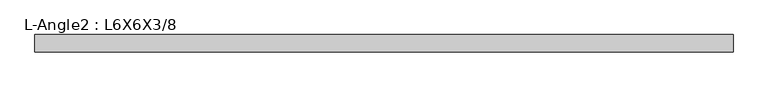
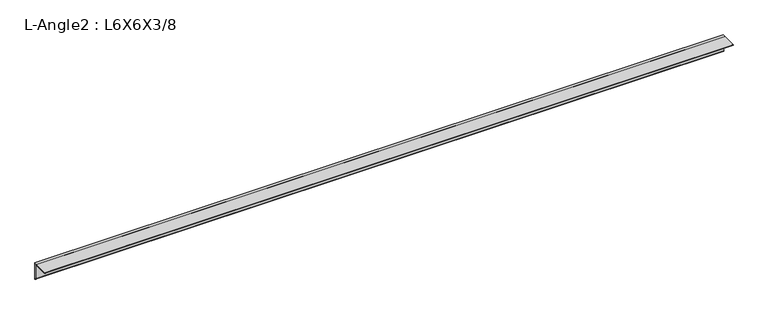
"""IFC4 building model written with IfcOpenShell, lengths in millimetres: member geometry, L-Angle2 : L6X6X3/8."""

import ifcopenshell
import ifcopenshell.guid

model = None  # the IFC model being written
_history = None  # IfcOwnerHistory: only IFC2X3 demands one
_inside = {}  # id of a spatial element -> (the spatial element, [elements in it])
_under = {}  # id of a project, library or spatial element -> (it, [spatial elements below it])
_declared = {}  # id of a project -> (the project, [libraries it declares])
_typed = {}  # id of a type object -> (the type object, [elements of that type])
_made_of = {}  # id of a material, layer set ... -> (it, [elements and type objects made of it])


def new_model(schema):
    """Start an empty IFC model of exactly this schema.

    Asked for "IFC4X3", IfcOpenShell would pick the latest addendum, in which some entities
    have other attributes; the version numbers below select the first issue.
    IFC2X3 requires an IfcOwnerHistory on every rooted entity: one is made here for all.
    """
    global model, _history
    if schema == "IFC4X3":
        model = ifcopenshell.file(schema_version=(4, 3, 0, 0))
    else:
        model = ifcopenshell.file(schema=schema)
    _inside.clear()
    _under.clear()
    _declared.clear()
    _typed.clear()
    _made_of.clear()
    _history = None
    if model.schema == "IFC2X3":
        org = make("IfcOrganization", Name="unknown")
        user = make(
            "IfcPersonAndOrganization",
            ThePerson=make("IfcPerson", FamilyName="unknown"),
            TheOrganization=org,
        )
        app = make(
            "IfcApplication",
            ApplicationDeveloper=org,
            Version="unknown",
            ApplicationFullName="unknown",
            ApplicationIdentifier="unknown",
        )
        _history = make(
            "IfcOwnerHistory",
            OwningUser=user,
            OwningApplication=app,
            ChangeAction="ADDED",
            CreationDate=0,
        )
    return model


def make(cls, **values):
    """One entity of the class cls with the attributes given. An attribute that is None is left unset."""
    return model.create_entity(
        cls, **{name: value for name, value in values.items() if value is not None}
    )


def rooted(cls, **values):
    """An entity with a GlobalId (a new one), such as an element, a storey or a relation."""
    return make(cls, GlobalId=ifcopenshell.guid.new(), OwnerHistory=_history, **values)


def si_unit(unit_type, name, prefix=None):
    """IfcSIUnit, for example si_unit("LENGTHUNIT", "METRE", prefix="MILLI")."""
    return make("IfcSIUnit", UnitType=unit_type, Prefix=prefix, Name=name)


def assignment(units):
    """IfcUnitAssignment: the units of a project."""
    return None if units is None else make("IfcUnitAssignment", Units=units)


def point(xyz):
    """IfcCartesianPoint."""
    return None if xyz is None else make("IfcCartesianPoint", Coordinates=xyz)


def direction(xyz):
    """IfcDirection."""
    return None if xyz is None else make("IfcDirection", DirectionRatios=xyz)


def frame(location, z_axis=None, x_axis=None):
    """IfcAxis2Placement3D, a coordinate frame: its origin and axes. An axis left out is left unset."""
    return make(
        "IfcAxis2Placement3D",
        Location=point(location),
        Axis=direction(z_axis),
        RefDirection=direction(x_axis),
    )


def frame_2d(location, x_axis=None):
    """IfcAxis2Placement2D, a coordinate frame in the plane: its origin and x axis."""
    return make(
        "IfcAxis2Placement2D", Location=point(location), RefDirection=direction(x_axis)
    )


def origin():
    """The frame at (0, 0, 0) with its axes left unset."""
    return frame((0.0, 0.0, 0.0))


def place(relative_to, where):
    """IfcLocalPlacement: puts the frame where relative to a parent placement (None: the world)."""
    return make(
        "IfcLocalPlacement", PlacementRelTo=relative_to, RelativePlacement=where
    )


def context(
    kind, dimensions, precision=None, world=None, true_north=None, identifier=None
):
    """IfcGeometricRepresentationContext, for example the 3D "Model" context."""
    return make(
        "IfcGeometricRepresentationContext",
        ContextIdentifier=identifier,
        ContextType=kind,
        CoordinateSpaceDimension=dimensions,
        Precision=precision,
        WorldCoordinateSystem=world,
        TrueNorth=true_north,
    )


def project(units=None, contexts=None):
    """IfcProject with its units and contexts."""
    return rooted(
        "IfcProject",
        Name="project",
        RepresentationContexts=contexts,
        UnitsInContext=assignment(units),
    )


def spatial(cls, under=None, at=None, **own):
    """A site, building, storey or space (cls), placed at a placement, below another one or the project."""
    s = rooted(cls, ObjectPlacement=at, **own)
    if under is not None:
        _under.setdefault(under.id(), (under, []))[1].append(s)
    return s


def polyline(points):
    """IfcPolyline through the points."""
    return make("IfcPolyline", Points=[point(p) for p in points])


def circle_curve(where, radius):
    """IfcCircle in the frame where."""
    return make("IfcCircle", Position=where, Radius=radius)


def trimmed(basis, trim1, trim2, sense, master):
    """IfcTrimmedCurve: the piece of a basis curve between two trims."""
    return make(
        "IfcTrimmedCurve",
        BasisCurve=basis,
        Trim1=trim1,
        Trim2=trim2,
        SenseAgreement=sense,
        MasterRepresentation=master,
    )


def segment(curve, same_sense, transition):
    """IfcCompositeCurveSegment."""
    return make(
        "IfcCompositeCurveSegment",
        Transition=transition,
        SameSense=same_sense,
        ParentCurve=curve,
    )


def composite_curve(segments, self_intersect=None):
    """IfcCompositeCurve: segments joined end to end."""
    return make("IfcCompositeCurve", Segments=segments, SelfIntersect=self_intersect)


def outline(outer, holes=None, kind="AREA"):
    """IfcArbitraryClosedProfileDef: a profile drawn as a closed curve; with holes, ...WithVoids."""
    if holes is None:
        return make("IfcArbitraryClosedProfileDef", ProfileType=kind, OuterCurve=outer)
    return make(
        "IfcArbitraryProfileDefWithVoids",
        ProfileType=kind,
        OuterCurve=outer,
        InnerCurves=holes,
    )


def extrude(swept, where, along, depth):
    """IfcExtrudedAreaSolid: the profile swept, set in the frame where, extruded along a direction by depth."""
    return make(
        "IfcExtrudedAreaSolid",
        SweptArea=swept,
        Position=where,
        ExtrudedDirection=direction(along),
        Depth=depth,
    )


def shape(context_of_items, identifier, shape_type, items):
    """IfcShapeRepresentation: the items that make up one representation, for example the "Body"."""
    return make(
        "IfcShapeRepresentation",
        ContextOfItems=context_of_items,
        RepresentationIdentifier=identifier,
        RepresentationType=shape_type,
        Items=items,
    )


def source(mapping_origin, context_of_items, identifier, shape_type, items):
    """IfcRepresentationMap: a shape defined once, which mapped items show again and again."""
    return make(
        "IfcRepresentationMap",
        MappingOrigin=mapping_origin,
        MappedRepresentation=shape(context_of_items, identifier, shape_type, items),
    )


def transform(
    local_origin,
    x_axis=None,
    y_axis=None,
    z_axis=None,
    scale=None,
    scale2=None,
    scale3=None,
    uniform=True,
):
    """IfcCartesianTransformationOperator3D, or its non-uniform kind. x_axis, y_axis, z_axis: its Axis1, 2, 3."""
    if uniform:
        return make(
            "IfcCartesianTransformationOperator3D",
            Axis1=direction(x_axis),
            Axis2=direction(y_axis),
            LocalOrigin=point(local_origin),
            Scale=scale,
            Axis3=direction(z_axis),
        )
    return make(
        "IfcCartesianTransformationOperator3DnonUniform",
        Axis1=direction(x_axis),
        Axis2=direction(y_axis),
        LocalOrigin=point(local_origin),
        Scale=scale,
        Axis3=direction(z_axis),
        Scale2=scale2,
        Scale3=scale3,
    )


def mapped(mapping_source, mapping_target):
    """IfcMappedItem: shows the shape of a source again, moved by a transform."""
    return make(
        "IfcMappedItem", MappingSource=mapping_source, MappingTarget=mapping_target
    )


def made_of(thing, what):
    """Note that an element or type object is made of a material, layer set ...; save() writes the relation."""
    if what is not None:
        _made_of.setdefault(what.id(), (what, []))[1].append(thing)
    return thing


def element(
    cls,
    number,
    at=None,
    inside=None,
    cuts=None,
    type_object=None,
    material=None,
    context=None,
    identifier="Body",
    shape_type=None,
    held_by="IfcProductDefinitionShape",
    body=None,
    shapes=None,
    **own,
):
    """One element of the class cls, such as IfcWall. Its Tag is "e" and its number.

    at: its placement. inside: the storey or other place that contains it. cuts: it is an
    opening in that element (IfcRelVoidsElement). A single representation is given by context,
    identifier, shape_type and body (its items); several are given by shapes. held_by: the class
    of the entity that holds the representations. save() writes the other relations.
    """
    e = rooted(cls, Tag="e%d" % number, ObjectPlacement=at, **own)
    if body is not None:
        shapes = [shape(context, identifier, shape_type, body)]
    if shapes is not None:
        e.Representation = make(held_by, Representations=shapes)
    if inside is not None:
        _inside.setdefault(inside.id(), (inside, []))[1].append(e)
    if cuts is not None:
        rooted(
            "IfcRelVoidsElement", RelatingBuildingElement=cuts, RelatedOpeningElement=e
        )
    if type_object is not None:
        _typed.setdefault(type_object.id(), (type_object, []))[1].append(e)
    return made_of(e, material)


def aggregate(whole, parts):
    """IfcRelAggregates: a whole, such as a stair, and the parts it consists of."""
    return rooted("IfcRelAggregates", RelatingObject=whole, RelatedObjects=parts)


def save(model, path):
    """Write the relations noted so far, then the file.

    IfcRelAggregates (storeys below a building ...), IfcRelContainedInSpatialStructure (elements
    in a storey), IfcRelDefinesByType, IfcRelAssociatesMaterial and IfcRelDeclares: one each for
    every whole, place, type object, material and project.
    """
    for whole, parts in _under.values():
        aggregate(whole, parts)
    for where, things in _inside.values():
        rooted(
            "IfcRelContainedInSpatialStructure",
            RelatedElements=things,
            RelatingStructure=where,
        )
    for kind, things in _typed.values():
        rooted("IfcRelDefinesByType", RelatedObjects=things, RelatingType=kind)
    for what, things in _made_of.values():
        rooted("IfcRelAssociatesMaterial", RelatedObjects=things, RelatingMaterial=what)
    for by, libraries in _declared.values():
        rooted("IfcRelDeclares", RelatingContext=by, RelatedDefinitions=libraries)
    model.write(path)


def l_angle2_l6x6x3_8_edb1527c(model_context):
    return source(origin(), model_context, "Body", "SweptSolid", [
        extrude(outline(composite_curve([segment(polyline([(41.148, 41.148), (41.148, -111.252)]), True, "CONTINUOUS"), segment(trimmed(circle_curve(frame_2d((41.148, -101.727)), 9.525), [point((41.148, -111.252))], [point((31.623, -101.727))], False, "CARTESIAN"), True, "CONTINUOUS"), segment(polyline([(31.623, -101.727), (31.623, 22.098)]), True, "CONTINUOUS"), segment(trimmed(circle_curve(frame_2d((22.098, 22.098)), 9.525), [point((31.623, 22.098))], [point((22.098, 31.623))], True, "CARTESIAN"), True, "CONTINUOUS"), segment(polyline([(22.098, 31.623), (-101.727, 31.623)]), True, "CONTINUOUS"), segment(trimmed(circle_curve(frame_2d((-101.727, 41.148)), 9.525), [point((-101.727, 31.623))], [point((-111.252, 41.148))], False, "CARTESIAN"), True, "CONTINUOUS"), segment(polyline([(-111.252, 41.148), (41.148, 41.148)]), True, "CONTINUOUS")], self_intersect=False)), frame((-3087.7876533, 0.0, 0.0), z_axis=(1.0, 0.0, 0.0), x_axis=(0.0, 1.0, 0.0)), (0.0, 0.0, 1.0), 6141.9768896),
    ])


if __name__ == "__main__":
    model = new_model("IFC4")
    model_context = context("Model", 3, world=origin())
    ifc_project = project(units=[si_unit("LENGTHUNIT", "METRE", prefix="MILLI")], contexts=[model_context])
    site = spatial("IfcSite", under=ifc_project)
    building = spatial("IfcBuilding", under=site)
    placement = place(None, origin())
    l_angle2_l6x6x3_8_shape = l_angle2_l6x6x3_8_edb1527c(model_context)
    element("IfcMember", 1, ObjectType="L-Angle2 : L6X6X3/8", at=placement, inside=building, context=model_context, shape_type="MappedRepresentation", body=[
        mapped(l_angle2_l6x6x3_8_shape, transform((0.0, 0.0, 0.0), x_axis=(1.0, 0.0, 0.0), y_axis=(0.0, 1.0, 0.0), z_axis=(0.0, 0.0, 1.0))),
    ])
    save(model, "model.ifc")

# Revit data of these elements
# Type "L-Angle2 : L6X6X3/8"
#   Assembly Code = "B10"
#   k = 0' - 0 7/8"
#   W = 14.9
#   Length [instance default] = 5' - 0"
#   b = 0' - 6"
#   d = 0' - 6"
#   t = 0' - 0 3/8"
#   x = 0' - 1.62"
#   y = 0' - 1.62"
#   A = 0.0304167 SF
#   Structural Material [instance default] = Steel ASTM A36
# Element 1 (IfcMember, "L-Angle2 : L6X6X3/8")
#   Materials on its faces: "Steel ASTM A36"
# Materials
#   "Steel ASTM A36": class "Metal", colour RGB 199 199 199, transparency 0, Description = "Structural steel, ASTM A36 Grade B, mill finish", Cost = 0
